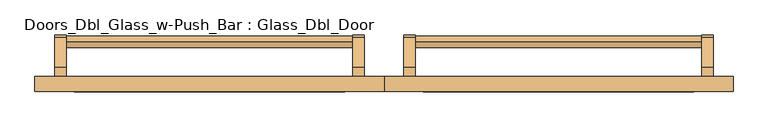
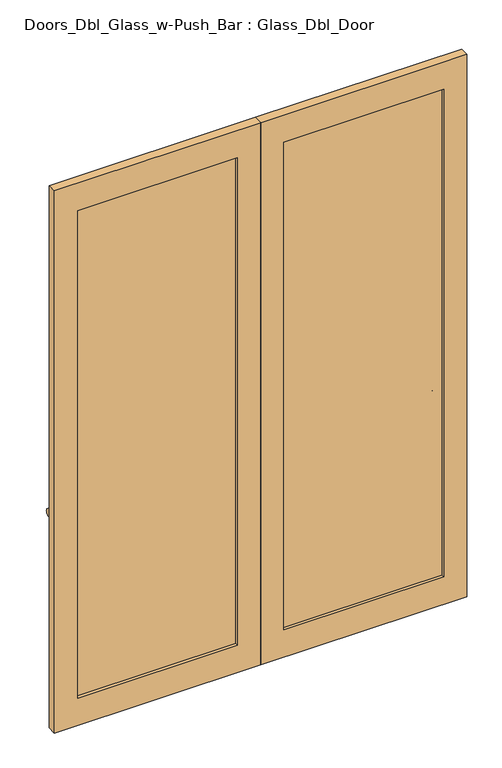
"""IFC4 building model written with IfcOpenShell, lengths in millimetres: door geometry, Doors_Dbl_Glass_w-Push_Bar : Glass_Dbl_Door."""

from ifc_helpers import new_model, si_unit, point, frame, frame_2d, origin, place, context, project, spatial, polyline, circle_curve, trimmed, segment, composite_curve, outline, extrude, source, transform, mapped, element, save


def doors_dbl_glass_w_push_bar_glass_dbl_door_09b0a2ef(model_context):
    return source(origin(), model_context, "Body", "SweptSolid", [
        extrude(outline(composite_curve([segment(trimmed(circle_curve(frame_2d((65.0203019, 909.5721086)), 15.0), [point((65.0203019, 924.5721086))], [point((65.0203019, 894.5721086))], False, "CARTESIAN"), True, "CONTINUOUS"), segment(trimmed(circle_curve(frame_2d((65.0203019, 909.5721086)), 15.0), [point((65.0203019, 894.5721086))], [point((65.0203019, 924.5721086))], False, "CARTESIAN"), True, "CONTINUOUS")], self_intersect=False)), frame((80.0, 0.0, 0.0), z_axis=(1.0, 0.0, 0.0), x_axis=(0.0, 1.0, 0.0)), (0.0, 0.0, 1.0), 730.0),
        extrude(outline(composite_curve([segment(polyline([(-0.1563269, 1000.0), (77.6459332, 922.19774)]), True, "CONTINUOUS"), segment(trimmed(circle_curve(frame_2d((65.0203019, 909.5721086)), 17.8553391), [point((77.6459332, 922.19774))], [point((52.3946705, 896.9464773))], False, "CARTESIAN"), True, "CONTINUOUS"), segment(polyline([(52.3946705, 896.9464773), (14.3411478, 935.0), (-24.035259, 935.0), (-24.035259, 1000.0), (-0.1563269, 1000.0)]), True, "CONTINUOUS")], self_intersect=False)), frame((810.0, 0.0, 0.0), z_axis=(1.0, 0.0, 0.0), x_axis=(0.0, 1.0, 0.0)), (0.0, 0.0, 1.0), 30.0),
        extrude(outline(composite_curve([segment(polyline([(-0.1563269, 1000.0), (77.6459332, 922.19774)]), True, "CONTINUOUS"), segment(trimmed(circle_curve(frame_2d((65.0203019, 909.5721086)), 17.8553391), [point((77.6459332, 922.19774))], [point((52.3946705, 896.9464773))], False, "CARTESIAN"), True, "CONTINUOUS"), segment(polyline([(52.3946705, 896.9464773), (14.3411478, 935.0), (-24.035259, 935.0), (-24.035259, 1000.0), (-0.1563269, 1000.0)]), True, "CONTINUOUS")], self_intersect=False)), frame((50.0, 0.0, 0.0), z_axis=(1.0, 0.0, 0.0), x_axis=(0.0, 1.0, 0.0)), (0.0, 0.0, 1.0), 30.0),
        extrude(outline(composite_curve([segment(trimmed(circle_curve(frame_2d((65.0203019, 909.5721086)), 15.0), [point((65.0203019, 924.5721086))], [point((65.0203019, 894.5721086))], False, "CARTESIAN"), True, "CONTINUOUS"), segment(trimmed(circle_curve(frame_2d((65.0203019, 909.5721086)), 15.0), [point((65.0203019, 894.5721086))], [point((65.0203019, 924.5721086))], False, "CARTESIAN"), True, "CONTINUOUS")], self_intersect=False)), frame((-810.0, 0.0, 0.0), z_axis=(1.0, 0.0, 0.0), x_axis=(0.0, 1.0, 0.0)), (0.0, 0.0, 1.0), 730.0),
        extrude(outline(composite_curve([segment(polyline([(-0.1563269, 1000.0), (77.6459332, 922.19774)]), True, "CONTINUOUS"), segment(trimmed(circle_curve(frame_2d((65.0203019, 909.5721086)), 17.8553391), [point((77.6459332, 922.19774))], [point((52.3946705, 896.9464773))], False, "CARTESIAN"), True, "CONTINUOUS"), segment(polyline([(52.3946705, 896.9464773), (14.3411478, 935.0), (-24.035259, 935.0), (-24.035259, 1000.0), (-0.1563269, 1000.0)]), True, "CONTINUOUS")], self_intersect=False)), frame((-80.0, 0.0, 0.0), z_axis=(1.0, 0.0, 0.0), x_axis=(0.0, 1.0, 0.0)), (0.0, 0.0, 1.0), 30.0),
        extrude(outline(composite_curve([segment(polyline([(-0.1563269, 1000.0), (77.6459332, 922.19774)]), True, "CONTINUOUS"), segment(trimmed(circle_curve(frame_2d((65.0203019, 909.5721086)), 17.8553391), [point((77.6459332, 922.19774))], [point((52.3946705, 896.9464773))], False, "CARTESIAN"), True, "CONTINUOUS"), segment(polyline([(52.3946705, 896.9464773), (14.3411478, 935.0), (-24.035259, 935.0), (-24.035259, 1000.0), (-0.1563269, 1000.0)]), True, "CONTINUOUS")], self_intersect=False)), frame((-840.0, 0.0, 0.0), z_axis=(1.0, 0.0, 0.0), x_axis=(0.0, 1.0, 0.0)), (0.0, 0.0, 1.0), 30.0),
        extrude(outline(polyline([(2475.0, -890.0), (0.0, -890.0), (0.0, 0.0), (2475.0, 0.0), (2475.0, -890.0)]), holes=[polyline([(2350.0, -790.0), (2350.0, -100.0), (125.0, -100.0), (125.0, -790.0), (2350.0, -790.0)])]), frame((0.0, -62.5788556, 0.0), z_axis=(0.0, 1.0, 0.0), x_axis=(0.0, 0.0, 1.0)), (0.0, 0.0, 1.0), 38.5435966),
        extrude(outline(polyline([(2475.0, 0.0), (0.0, 0.0), (0.0, 890.0), (2475.0, 890.0), (2475.0, 0.0)]), holes=[polyline([(2350.0, 100.0), (2350.0, 790.0), (125.0, 790.0), (125.0, 100.0), (2350.0, 100.0)])]), frame((0.0, -62.5788556, 0.0), z_axis=(0.0, 1.0, 0.0), x_axis=(0.0, 0.0, 1.0)), (0.0, 0.0, 1.0), 38.5435966),
        extrude(outline(polyline([(-100.0, -38.0), (-100.0, -50.0), (-790.0, -50.0), (-790.0, -38.0), (-100.0, -38.0)])), frame((0.0, 0.0, 125.0), z_axis=(0.0, 0.0, 1.0), x_axis=(1.0, 0.0, 0.0)), (0.0, 0.0, 1.0), 2225.0),
        extrude(outline(polyline([(790.0, -38.0), (790.0, -50.0), (100.0, -50.0), (100.0, -38.0), (790.0, -38.0)])), frame((0.0, 0.0, 125.0), z_axis=(0.0, 0.0, 1.0), x_axis=(1.0, 0.0, 0.0)), (0.0, 0.0, 1.0), 2225.0),
    ])


if __name__ == "__main__":
    model = new_model("IFC4")
    model_context = context("Model", 3, world=origin())
    ifc_project = project(units=[si_unit("LENGTHUNIT", "METRE", prefix="MILLI")], contexts=[model_context])
    site = spatial("IfcSite", under=ifc_project)
    building = spatial("IfcBuilding", under=site)
    placement = place(None, origin())
    doors_dbl_glass_w_push_bar_glass_dbl_door_shape = doors_dbl_glass_w_push_bar_glass_dbl_door_09b0a2ef(model_context)
    element("IfcDoor", 1, ObjectType="Doors_Dbl_Glass_w-Push_Bar : Glass_Dbl_Door", at=placement, inside=building, context=model_context, shape_type="MappedRepresentation", body=[
        mapped(doors_dbl_glass_w_push_bar_glass_dbl_door_shape, transform((0.0, 0.0, 0.0), x_axis=(1.0, 0.0, 0.0), y_axis=(0.0, 1.0, 0.0), z_axis=(0.0, 0.0, 1.0))),
    ])
    save(model, "model.ifc")

# Revit data of these elements
# Type "Doors_Dbl_Glass_w-Push_Bar : Glass_Dbl_Door"
#   Type Mark = "46"
#   Construction Type Id = "GSP4R"
#   Analytic Construction = "1/8 in Pilkington single glazing"
#   Visual Light Transmittance = 0.9
#   TopRail = 125 mm
#   Solar Heat Gain Coefficient = 0.78
#   Offset = 50 mm
#   MuntinRail = 100 mm
#   LockRail = 100 mm
#   Heat Transfer Coefficient (U) = 3.6886 W/(m²·K)
#   Handle Z Distance = 1000 mm
#   Handle X Offset = 65 mm
#   Glass Thickness = 12 mm
#   BottomRail = 125 mm
#   Material Ironmongery = Metal - Aluminum
#   Material Door = Metal - Aluminum
#   Material Glass = Glass
#   Function = (empty or 0)
# Element 1 (IfcDoor, "Doors_Dbl_Glass_w-Push_Bar : Glass_Dbl_Door")
#   Materials on its faces: "Metal - Aluminum", "Glass"
# Materials
#   "Metal - Aluminum": class "Metal", colour RGB 247 247 247, transparency 0
#   "Glass": class "Glass", colour RGB 0 128 192, transparency 0.9, Description = "Soda Lime Glass", Cost = 0
